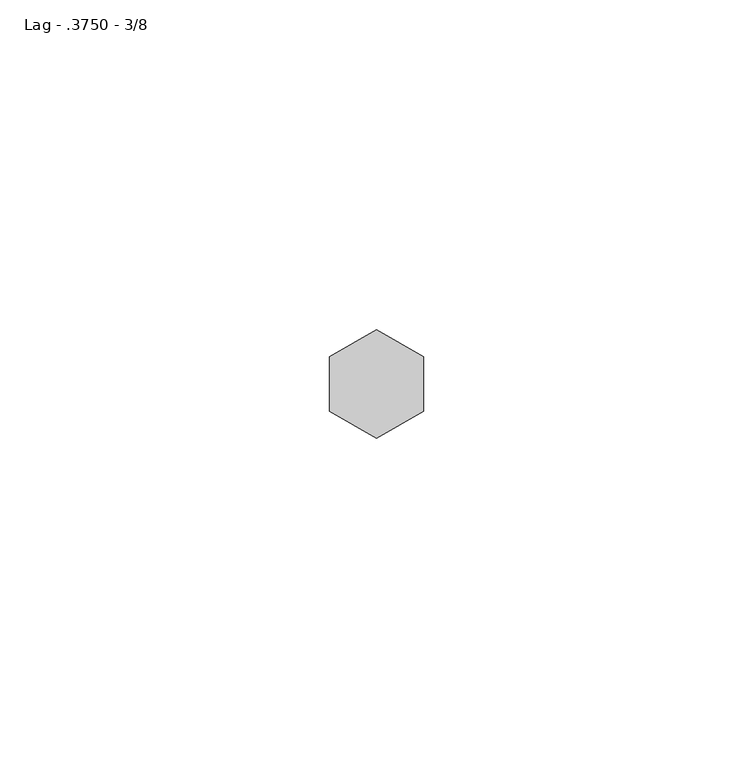
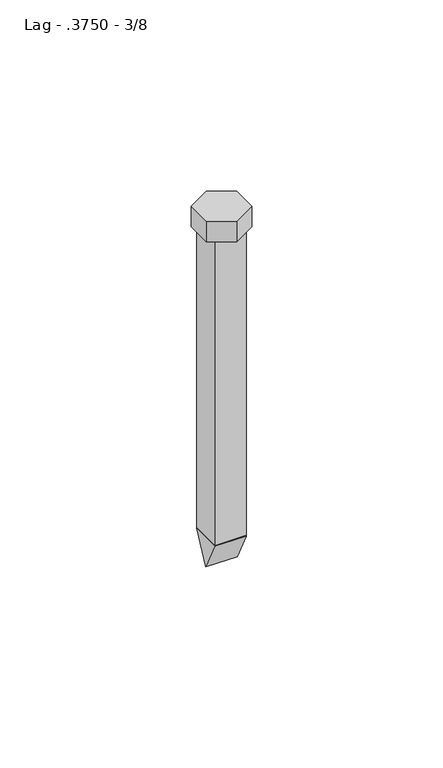
"""IFC4 building model written with IfcOpenShell, lengths in millimetres: fastener geometry, 060523 - W_P_C - Fastenings - Generic - SQUARE : Lag - .3750 - 3/8."""

from ifc_helpers import new_model, si_unit, frame, origin, origin_with_axes, place, context, project, spatial, polyline, outline, extrude, source, transform, mapped, element, save


def lag_3750_3_8_8cade9c9(model_context):
    return source(origin(), model_context, "Body", "SweptSolid", [
        extrude(outline(polyline([(0.0, -111.4226562), (-4.9113281, -101.6), (4.9113281, -101.6), (0.0, -111.4226562)])), frame((-4.9113281, 0.0, 0.0), z_axis=(1.0, 0.0, 0.0), x_axis=(0.0, 1.0, 0.0)), (0.0, 0.0, 1.0), 9.8226563),
        extrude(outline(polyline([(-7.14375, 4.124446), (0.0, 8.248892), (7.14375, 4.124446), (7.14375, -4.124446), (0.0, -8.248892), (-7.14375, -4.124446), (-7.14375, 4.124446)])), origin_with_axes(), (0.0, 0.0, 1.0), 6.8072),
        extrude(outline(polyline([(-4.9113281, 4.9113281), (4.9113281, 4.9113281), (4.9113281, -4.9113281), (-4.9113281, -4.9113281), (-4.9113281, 4.9113281)])), frame((0.0, 0.0, -101.6), z_axis=(0.0, 0.0, 1.0), x_axis=(1.0, 0.0, 0.0)), (0.0, 0.0, 1.0), 101.6),
    ])


if __name__ == "__main__":
    model = new_model("IFC4")
    model_context = context("Model", 3, world=origin())
    ifc_project = project(units=[si_unit("LENGTHUNIT", "METRE", prefix="MILLI")], contexts=[model_context])
    site = spatial("IfcSite", under=ifc_project)
    building = spatial("IfcBuilding", under=site)
    placement = place(None, origin())
    lag_3750_3_8_shape = lag_3750_3_8_8cade9c9(model_context)
    element("IfcFastener", 1, ObjectType="060523 - W_P_C - Fastenings - Generic - SQUARE : Lag - .3750 - 3/8", at=placement, inside=building, context=model_context, shape_type="MappedRepresentation", body=[
        mapped(lag_3750_3_8_shape, transform((0.0, 0.0, 0.0), x_axis=(1.0, 0.0, 0.0), y_axis=(0.0, 1.0, 0.0), z_axis=(0.0, 0.0, 1.0))),
    ])
    save(model, "model.ifc")

# Revit data of these elements
# Type "060523 - W_P_C - Fastenings - Generic - SQUARE : Lag - .3750 - 3/8"
#   Washer_Thickness = 0' - 0.08933"
#   Washer Radius = 0' - 0.46136"
#   Washer Offset - Head = 0' - 0"
#   Washer Offset = 0' - 0"
#   Thickness_of_Substrate [instance default] = 0' - 1"
#   Side = 0' - 0.3252"
#   Radius = 0' - 0.19336"
#   Length [instance default] = 0' - 4"
#   Head Size = 0' - 0 9/16"
#   Head Radius = 0' - 0 9/32"
#   Head Height = 0' - 0.268"
#   Double Diameter = 0' - 0 99/128"
#   Diameter = 0' - 0 99/256"
#   Default Elevation = 4' - 0"
#   Washer_Nut_Visibility = no
#   Washer_Head_Visibility = no
#   Round_Head_Visibility = no
#   Point Visibility = yes
#   Nut_Visibility = no
#   Hex_Head_Visiblilty = yes
#   Washer Material = none
#   Bolt Material (Size) = AT SILL - FASTENER AT 24" O.C.
# Element 1 (IfcFastener, "060523 - W_P_C - Fastenings - Generic - SQUARE : Lag - .3750 - 3/8")
#   Materials on its faces: "AT SILL - FASTENER AT 24\" O.C."
# Materials
#   "AT SILL - FASTENER AT 24\" O.C.": class "Generic", colour RGB 120 120 120, transparency 0, Cost = 0
